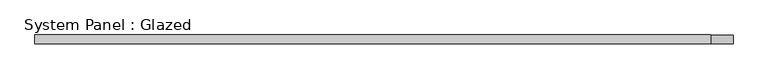
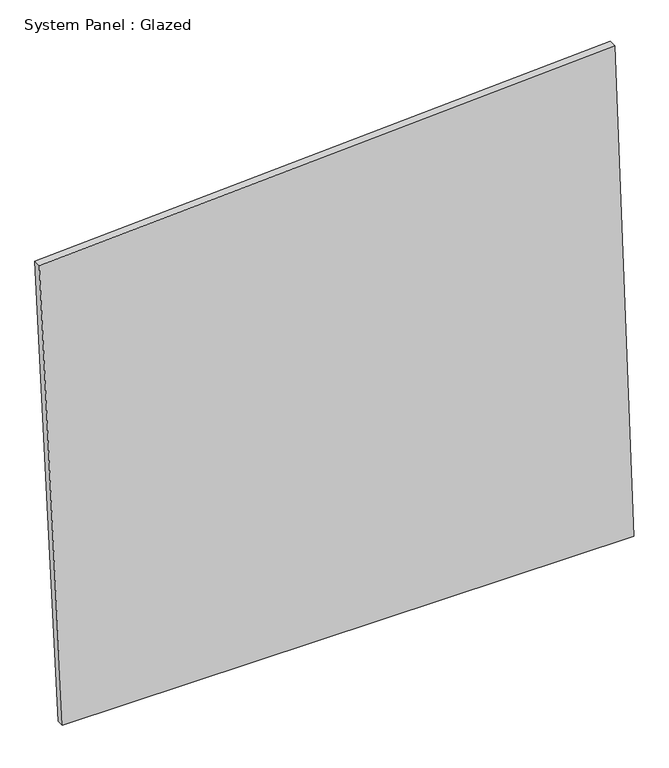
"""IFC4 building model written with IfcOpenShell, lengths in millimetres: plate geometry, System Panel : Glazed."""

from ifc_helpers import new_model, si_unit, frame, origin, place, context, project, spatial, polyline, outline, extrude, source, transform, mapped, element, save


def system_panel_glazed_61bd3bb4(model_context):
    return source(origin(), model_context, "Body", "SweptSolid", [
        extrude(outline(polyline([(0.0, -918.1552821), (0.0, 996.0695243), (1761.0937074, 931.9438881), (1655.9323013, -996.0695243), (0.0, -918.1552821)])), frame((0.0, -49.5, 0.0), z_axis=(0.0, 1.0, 0.0), x_axis=(0.0, 0.0, 1.0)), (0.0, 0.0, 1.0), 25.0),
    ])


if __name__ == "__main__":
    model = new_model("IFC4")
    model_context = context("Model", 3, world=origin())
    ifc_project = project(units=[si_unit("LENGTHUNIT", "METRE", prefix="MILLI")], contexts=[model_context])
    site = spatial("IfcSite", under=ifc_project)
    building = spatial("IfcBuilding", under=site)
    placement = place(None, origin())
    system_panel_glazed_shape = system_panel_glazed_61bd3bb4(model_context)
    element("IfcPlate", 1, ObjectType="System Panel : Glazed", at=placement, inside=building, context=model_context, shape_type="MappedRepresentation", body=[
        mapped(system_panel_glazed_shape, transform((0.0, 0.0, 0.0), x_axis=(1.0, 0.0, 0.0), y_axis=(0.0, 1.0, 0.0), z_axis=(0.0, 0.0, 1.0))),
    ])
    save(model, "model.ifc")

# Revit data of these elements
# Element 1 (IfcPlate, "System Panel : Glazed")
#   Materials on its faces: "Glass, Clear Glazing"
# Materials
#   "Glass, Clear Glazing": class "Glass", colour RGB 247 249 248, transparency 0.85, Description = "Clear glazing", Cost = 0
